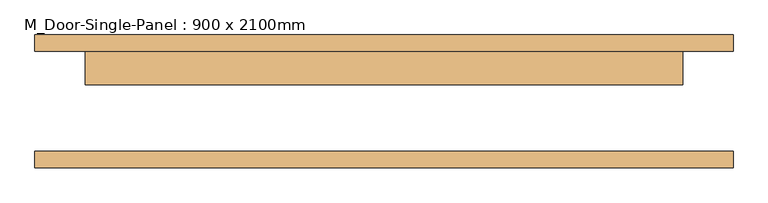
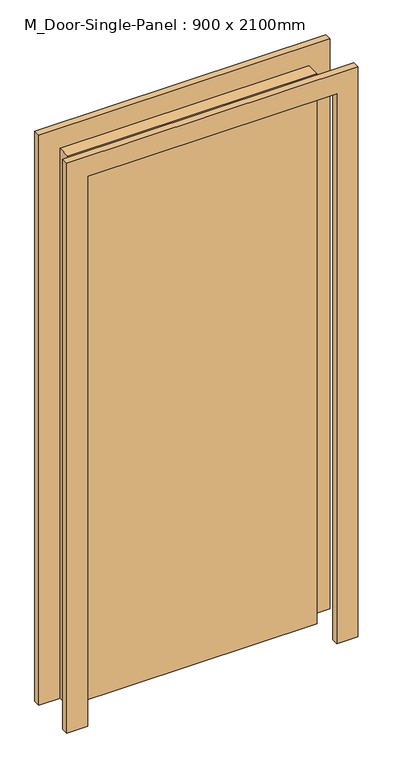
"""IFC4 building model written with IfcOpenShell, lengths in millimetres: door geometry, M_Door-Single-Panel : 900 x 2100mm."""

import ifcopenshell
import ifcopenshell.guid

model = None  # the IFC model being written
_history = None  # IfcOwnerHistory: only IFC2X3 demands one
_inside = {}  # id of a spatial element -> (the spatial element, [elements in it])
_under = {}  # id of a project, library or spatial element -> (it, [spatial elements below it])
_declared = {}  # id of a project -> (the project, [libraries it declares])
_typed = {}  # id of a type object -> (the type object, [elements of that type])
_made_of = {}  # id of a material, layer set ... -> (it, [elements and type objects made of it])


def new_model(schema):
    """Start an empty IFC model of exactly this schema.

    Asked for "IFC4X3", IfcOpenShell would pick the latest addendum, in which some entities
    have other attributes; the version numbers below select the first issue.
    IFC2X3 requires an IfcOwnerHistory on every rooted entity: one is made here for all.
    """
    global model, _history
    if schema == "IFC4X3":
        model = ifcopenshell.file(schema_version=(4, 3, 0, 0))
    else:
        model = ifcopenshell.file(schema=schema)
    _inside.clear()
    _under.clear()
    _declared.clear()
    _typed.clear()
    _made_of.clear()
    _history = None
    if model.schema == "IFC2X3":
        org = make("IfcOrganization", Name="unknown")
        user = make(
            "IfcPersonAndOrganization",
            ThePerson=make("IfcPerson", FamilyName="unknown"),
            TheOrganization=org,
        )
        app = make(
            "IfcApplication",
            ApplicationDeveloper=org,
            Version="unknown",
            ApplicationFullName="unknown",
            ApplicationIdentifier="unknown",
        )
        _history = make(
            "IfcOwnerHistory",
            OwningUser=user,
            OwningApplication=app,
            ChangeAction="ADDED",
            CreationDate=0,
        )
    return model


def make(cls, **values):
    """One entity of the class cls with the attributes given. An attribute that is None is left unset."""
    return model.create_entity(
        cls, **{name: value for name, value in values.items() if value is not None}
    )


def rooted(cls, **values):
    """An entity with a GlobalId (a new one), such as an element, a storey or a relation."""
    return make(cls, GlobalId=ifcopenshell.guid.new(), OwnerHistory=_history, **values)


def si_unit(unit_type, name, prefix=None):
    """IfcSIUnit, for example si_unit("LENGTHUNIT", "METRE", prefix="MILLI")."""
    return make("IfcSIUnit", UnitType=unit_type, Prefix=prefix, Name=name)


def assignment(units):
    """IfcUnitAssignment: the units of a project."""
    return None if units is None else make("IfcUnitAssignment", Units=units)


def point(xyz):
    """IfcCartesianPoint."""
    return None if xyz is None else make("IfcCartesianPoint", Coordinates=xyz)


def direction(xyz):
    """IfcDirection."""
    return None if xyz is None else make("IfcDirection", DirectionRatios=xyz)


def frame(location, z_axis=None, x_axis=None):
    """IfcAxis2Placement3D, a coordinate frame: its origin and axes. An axis left out is left unset."""
    return make(
        "IfcAxis2Placement3D",
        Location=point(location),
        Axis=direction(z_axis),
        RefDirection=direction(x_axis),
    )


def origin():
    """The frame at (0, 0, 0) with its axes left unset."""
    return frame((0.0, 0.0, 0.0))


def origin_with_axes():
    """The frame at (0, 0, 0) with the z axis (0, 0, 1) and the x axis (1, 0, 0) written out."""
    return frame((0.0, 0.0, 0.0), z_axis=(0.0, 0.0, 1.0), x_axis=(1.0, 0.0, 0.0))


def place(relative_to, where):
    """IfcLocalPlacement: puts the frame where relative to a parent placement (None: the world)."""
    return make(
        "IfcLocalPlacement", PlacementRelTo=relative_to, RelativePlacement=where
    )


def context(
    kind, dimensions, precision=None, world=None, true_north=None, identifier=None
):
    """IfcGeometricRepresentationContext, for example the 3D "Model" context."""
    return make(
        "IfcGeometricRepresentationContext",
        ContextIdentifier=identifier,
        ContextType=kind,
        CoordinateSpaceDimension=dimensions,
        Precision=precision,
        WorldCoordinateSystem=world,
        TrueNorth=true_north,
    )


def project(units=None, contexts=None):
    """IfcProject with its units and contexts."""
    return rooted(
        "IfcProject",
        Name="project",
        RepresentationContexts=contexts,
        UnitsInContext=assignment(units),
    )


def spatial(cls, under=None, at=None, **own):
    """A site, building, storey or space (cls), placed at a placement, below another one or the project."""
    s = rooted(cls, ObjectPlacement=at, **own)
    if under is not None:
        _under.setdefault(under.id(), (under, []))[1].append(s)
    return s


def polyline(points):
    """IfcPolyline through the points."""
    return make("IfcPolyline", Points=[point(p) for p in points])


def outline(outer, holes=None, kind="AREA"):
    """IfcArbitraryClosedProfileDef: a profile drawn as a closed curve; with holes, ...WithVoids."""
    if holes is None:
        return make("IfcArbitraryClosedProfileDef", ProfileType=kind, OuterCurve=outer)
    return make(
        "IfcArbitraryProfileDefWithVoids",
        ProfileType=kind,
        OuterCurve=outer,
        InnerCurves=holes,
    )


def extrude(swept, where, along, depth):
    """IfcExtrudedAreaSolid: the profile swept, set in the frame where, extruded along a direction by depth."""
    return make(
        "IfcExtrudedAreaSolid",
        SweptArea=swept,
        Position=where,
        ExtrudedDirection=direction(along),
        Depth=depth,
    )


def shape(context_of_items, identifier, shape_type, items):
    """IfcShapeRepresentation: the items that make up one representation, for example the "Body"."""
    return make(
        "IfcShapeRepresentation",
        ContextOfItems=context_of_items,
        RepresentationIdentifier=identifier,
        RepresentationType=shape_type,
        Items=items,
    )


def source(mapping_origin, context_of_items, identifier, shape_type, items):
    """IfcRepresentationMap: a shape defined once, which mapped items show again and again."""
    return make(
        "IfcRepresentationMap",
        MappingOrigin=mapping_origin,
        MappedRepresentation=shape(context_of_items, identifier, shape_type, items),
    )


def transform(
    local_origin,
    x_axis=None,
    y_axis=None,
    z_axis=None,
    scale=None,
    scale2=None,
    scale3=None,
    uniform=True,
):
    """IfcCartesianTransformationOperator3D, or its non-uniform kind. x_axis, y_axis, z_axis: its Axis1, 2, 3."""
    if uniform:
        return make(
            "IfcCartesianTransformationOperator3D",
            Axis1=direction(x_axis),
            Axis2=direction(y_axis),
            LocalOrigin=point(local_origin),
            Scale=scale,
            Axis3=direction(z_axis),
        )
    return make(
        "IfcCartesianTransformationOperator3DnonUniform",
        Axis1=direction(x_axis),
        Axis2=direction(y_axis),
        LocalOrigin=point(local_origin),
        Scale=scale,
        Axis3=direction(z_axis),
        Scale2=scale2,
        Scale3=scale3,
    )


def mapped(mapping_source, mapping_target):
    """IfcMappedItem: shows the shape of a source again, moved by a transform."""
    return make(
        "IfcMappedItem", MappingSource=mapping_source, MappingTarget=mapping_target
    )


def made_of(thing, what):
    """Note that an element or type object is made of a material, layer set ...; save() writes the relation."""
    if what is not None:
        _made_of.setdefault(what.id(), (what, []))[1].append(thing)
    return thing


def element(
    cls,
    number,
    at=None,
    inside=None,
    cuts=None,
    type_object=None,
    material=None,
    context=None,
    identifier="Body",
    shape_type=None,
    held_by="IfcProductDefinitionShape",
    body=None,
    shapes=None,
    **own,
):
    """One element of the class cls, such as IfcWall. Its Tag is "e" and its number.

    at: its placement. inside: the storey or other place that contains it. cuts: it is an
    opening in that element (IfcRelVoidsElement). A single representation is given by context,
    identifier, shape_type and body (its items); several are given by shapes. held_by: the class
    of the entity that holds the representations. save() writes the other relations.
    """
    e = rooted(cls, Tag="e%d" % number, ObjectPlacement=at, **own)
    if body is not None:
        shapes = [shape(context, identifier, shape_type, body)]
    if shapes is not None:
        e.Representation = make(held_by, Representations=shapes)
    if inside is not None:
        _inside.setdefault(inside.id(), (inside, []))[1].append(e)
    if cuts is not None:
        rooted(
            "IfcRelVoidsElement", RelatingBuildingElement=cuts, RelatedOpeningElement=e
        )
    if type_object is not None:
        _typed.setdefault(type_object.id(), (type_object, []))[1].append(e)
    return made_of(e, material)


def aggregate(whole, parts):
    """IfcRelAggregates: a whole, such as a stair, and the parts it consists of."""
    return rooted("IfcRelAggregates", RelatingObject=whole, RelatedObjects=parts)


def save(model, path):
    """Write the relations noted so far, then the file.

    IfcRelAggregates (storeys below a building ...), IfcRelContainedInSpatialStructure (elements
    in a storey), IfcRelDefinesByType, IfcRelAssociatesMaterial and IfcRelDeclares: one each for
    every whole, place, type object, material and project.
    """
    for whole, parts in _under.values():
        aggregate(whole, parts)
    for where, things in _inside.values():
        rooted(
            "IfcRelContainedInSpatialStructure",
            RelatedElements=things,
            RelatingStructure=where,
        )
    for kind, things in _typed.values():
        rooted("IfcRelDefinesByType", RelatedObjects=things, RelatingType=kind)
    for what, things in _made_of.values():
        rooted("IfcRelAssociatesMaterial", RelatedObjects=things, RelatingMaterial=what)
    for by, libraries in _declared.values():
        rooted("IfcRelDeclares", RelatingContext=by, RelatedDefinitions=libraries)
    model.write(path)


def m_door_single_panel_900_x_2100mm_302ab5a4(model_context):
    return source(origin(), model_context, "Body", "SweptSolid", [
        extrude(outline(polyline([(450.0, 25.0), (-450.0, 25.0), (-450.0, 75.0), (450.0, 75.0), (450.0, 25.0)])), origin_with_axes(), (0.0, 0.0, 1.0), 2100.0),
        extrude(outline(polyline([(2176.2, 526.2), (2176.2, -526.2), (0.0, -526.2), (0.0, -450.0), (2100.0, -450.0), (2100.0, 450.0), (0.0, 450.0), (0.0, 526.2), (2176.2, 526.2)])), frame((0.0, -100.0, 0.0), z_axis=(0.0, 1.0, 0.0), x_axis=(0.0, 0.0, 1.0)), (0.0, 0.0, 1.0), 25.0),
        extrude(outline(polyline([(2176.2, -526.2), (0.0, -526.2), (0.0, -450.0), (2100.0, -450.0), (2100.0, 450.0), (0.0, 450.0), (0.0, 526.2), (2176.2, 526.2), (2176.2, -526.2)])), frame((0.0, 75.0, 0.0), z_axis=(0.0, 1.0, 0.0), x_axis=(0.0, 0.0, 1.0)), (0.0, 0.0, 1.0), 25.0),
    ])


if __name__ == "__main__":
    model = new_model("IFC4")
    model_context = context("Model", 3, world=origin())
    ifc_project = project(units=[si_unit("LENGTHUNIT", "METRE", prefix="MILLI")], contexts=[model_context])
    site = spatial("IfcSite", under=ifc_project)
    building = spatial("IfcBuilding", under=site)
    placement = place(None, origin())
    m_door_single_panel_900_x_2100mm_shape = m_door_single_panel_900_x_2100mm_302ab5a4(model_context)
    element("IfcDoor", 1, ObjectType="M_Door-Single-Panel : 900 x 2100mm", at=placement, inside=building, context=model_context, shape_type="MappedRepresentation", body=[
        mapped(m_door_single_panel_900_x_2100mm_shape, transform((0.0, 0.0, 0.0), x_axis=(1.0, 0.0, 0.0), y_axis=(0.0, 1.0, 0.0), z_axis=(0.0, 0.0, 1.0))),
    ])
    save(model, "model.ifc")

# Revit data of these elements
# Type "M_Door-Single-Panel : 900 x 2100mm"
#   Type Mark = "48"
#   Construction Type Id = "DOOR"
#   Analytic Construction = "Wooden"
#   Thickness = 0.05 m
#   Thermal Resistance (R) = 0.455703 (m²·K)/W
#   Swing Angle [instance default] = 90.00°
#   Heat Transfer Coefficient (U) = 2.19465 W/(m²·K)
#   Height = 2.10 m
#   Trim Projection Ext = 0.025 m
#   Trim Projection Int = 0.025 m
#   Trim Width = 0.08 m
#   Width = 0.90 m
#   Define Thermal Properties by = 1
#   Panel Material = Wood - Birch - Solid Stained Light Low Gloss
#   Trim Material = Paint - Sienna
#   Visual Light Transmittance = 0
#   Solar Heat Gain Coefficient = 0
#   Function = (empty or 0)
#   Wall Closure = (empty or 0)
# Element 1 (IfcDoor, "M_Door-Single-Panel : 900 x 2100mm")
#   Materials on its faces: "Paint - Sienna", "Wood - Birch - Solid Stained Light Low Gloss"
# Materials
#   "Wood - Birch - Solid Stained Light Low Gloss": class "Wood", colour RGB 210 159 95, transparency 0, Cost = 0
#   "Paint - Sienna": class "Miscellaneous", colour RGB 118 70 51, transparency 0, Cost = 0
